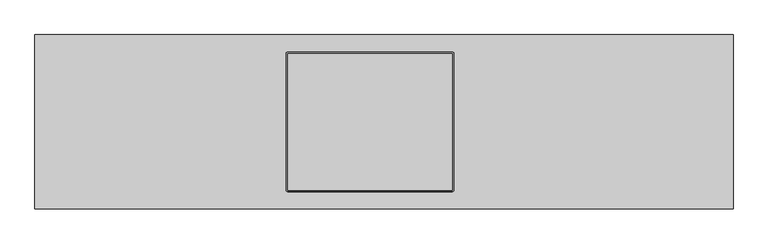
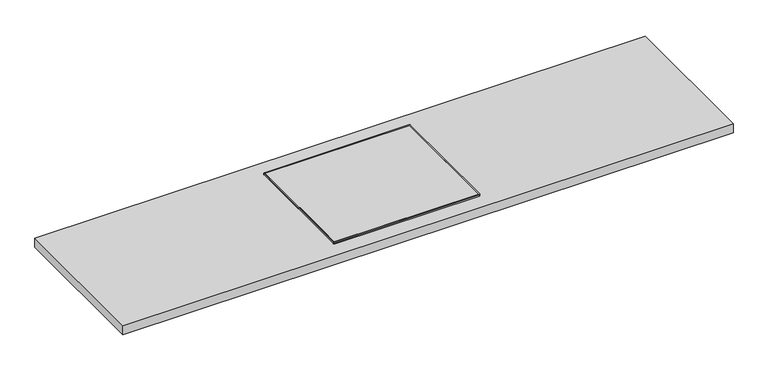
"""IFC4 building model written with IfcOpenShell, lengths in millimetres: furniture geometry, Arbeitsplatte - Mit Kochfeld : 600 mm Tiefe."""

from ifc_helpers import new_model, si_unit, point, frame, frame_2d, origin, place, context, project, spatial, polyline, circle_curve, trimmed, segment, composite_curve, outline, extrude, source, transform, mapped, element, save


def furniture_a2ae4300(model_context):
    return source(origin(), model_context, "Body", "SweptSolid", [
        extrude(outline(polyline([(294.5377049, -67.5), (294.5377049, -557.5), (-295.4622951, -557.5), (-295.4622951, -67.5), (294.5377049, -67.5)])), frame((0.0, 0.0, 900.0), z_axis=(0.0, 0.0, 1.0), x_axis=(1.0, 0.0, 0.0)), (0.0, 0.0, 1.0), 5.0),
        extrude(outline(composite_curve([segment(polyline([(-300.4622951, -557.5), (-300.4622951, -67.5)]), True, "CONTINUOUS"), segment(trimmed(circle_curve(frame_2d((-295.4622951, -67.5)), 5.0), [point((-300.4622951, -67.5))], [point((-295.4622951, -62.5))], False, "CARTESIAN"), True, "CONTINUOUS"), segment(polyline([(-295.4622951, -62.5), (294.5377049, -62.5)]), True, "CONTINUOUS"), segment(trimmed(circle_curve(frame_2d((294.5377049, -67.5)), 5.0), [point((294.5377049, -62.5))], [point((299.5377049, -67.5))], False, "CARTESIAN"), True, "CONTINUOUS"), segment(polyline([(299.5377049, -67.5), (299.5377049, -557.5)]), True, "CONTINUOUS"), segment(trimmed(circle_curve(frame_2d((294.5377049, -557.5)), 5.0), [point((299.5377049, -557.5))], [point((294.5377049, -562.5))], False, "CARTESIAN"), True, "CONTINUOUS"), segment(polyline([(294.5377049, -562.5), (-295.4622951, -562.5)]), True, "CONTINUOUS"), segment(trimmed(circle_curve(frame_2d((-295.4622951, -557.5)), 5.0), [point((-295.4622951, -562.5))], [point((-300.4622951, -557.5))], False, "CARTESIAN"), True, "CONTINUOUS")], self_intersect=False), holes=[polyline([(294.5377049, -67.5), (-295.4622951, -67.5), (-295.4622951, -557.5), (294.5377049, -557.5), (294.5377049, -67.5)])]), frame((0.0, 0.0, 900.0), z_axis=(0.0, 0.0, 1.0), x_axis=(1.0, 0.0, 0.0)), (0.0, 0.0, 1.0), 5.0),
        extrude(outline(polyline([(1299.5377049, 0.0), (1299.5377049, -625.0), (-1200.4622951, -625.0), (-1200.4622951, 0.0), (1299.5377049, 0.0)]), holes=[composite_curve([segment(polyline([(294.5377049, -62.5), (-295.4622951, -62.5)]), True, "CONTINUOUS"), segment(trimmed(circle_curve(frame_2d((-295.4622951, -67.5)), 5.0), [point((-295.4622951, -62.5))], [point((-300.4622951, -67.5))], True, "CARTESIAN"), True, "CONTINUOUS"), segment(polyline([(-300.4622951, -67.5), (-300.4622951, -557.5)]), True, "CONTINUOUS"), segment(trimmed(circle_curve(frame_2d((-295.4622951, -557.5)), 5.0), [point((-300.4622951, -557.5))], [point((-295.4622951, -562.5))], True, "CARTESIAN"), True, "CONTINUOUS"), segment(polyline([(-295.4622951, -562.5), (294.5377049, -562.5)]), True, "CONTINUOUS"), segment(trimmed(circle_curve(frame_2d((294.5377049, -557.5)), 5.0), [point((294.5377049, -562.5))], [point((299.5377049, -557.5))], True, "CARTESIAN"), True, "CONTINUOUS"), segment(polyline([(299.5377049, -557.5), (299.5377049, -67.5)]), True, "CONTINUOUS"), segment(trimmed(circle_curve(frame_2d((294.5377049, -67.5)), 5.0), [point((299.5377049, -67.5))], [point((294.5377049, -62.5))], True, "CARTESIAN"), True, "CONTINUOUS")], self_intersect=False)]), frame((0.0, 0.0, 860.0), z_axis=(0.0, 0.0, 1.0), x_axis=(1.0, 0.0, 0.0)), (0.0, 0.0, 1.0), 40.0),
    ])


if __name__ == "__main__":
    model = new_model("IFC4")
    model_context = context("Model", 3, world=origin())
    ifc_project = project(units=[si_unit("LENGTHUNIT", "METRE", prefix="MILLI")], contexts=[model_context])
    site = spatial("IfcSite", under=ifc_project)
    building = spatial("IfcBuilding", under=site)
    placement = place(None, origin())
    furniture_shape = furniture_a2ae4300(model_context)
    element("IfcFurniture", 1, ObjectType="Arbeitsplatte - Mit Kochfeld : 600 mm Tiefe", at=placement, inside=building, context=model_context, shape_type="MappedRepresentation", body=[
        mapped(furniture_shape, transform((0.0, 0.0, 0.0), x_axis=(1.0, 0.0, 0.0), y_axis=(0.0, 1.0, 0.0), z_axis=(0.0, 0.0, 1.0))),
    ])
    save(model, "model.ifc")

# Revit data of these elements
# Type "Arbeitsplatte - Mit Kochfeld : 600 mm Tiefe"
#   Dicke = 0.040 m
#   Depth = 0.625 m
#   Height = 0.900 m
#   Länge [instance default] = 2.500 m
#   Seitlicher Versatz Kochfeld [instance default] = 1.200 m
#   Tiefe Kochfeld [instance default] = 0.500 m
#   Breite Kochfeld [instance default] = 0.600 m
#   Rahmen Kochfeld = Metall - Aluminium
#   Kochfeld = Metall - Grau
#   Arbeitsplatte = Metall - Aluminium
# Element 1 (IfcFurniture, "Arbeitsplatte - Mit Kochfeld : 600 mm Tiefe")
#   Materials on its faces: "Metall - Aluminium", "Metall - Grau"
# Materials
#   "Metall - Aluminium": class "Metall", colour RGB 247 247 247, transparency 0, Description = "Aluminium 6061", Cost = 0
#   "Metall - Grau": class "Metall", colour RGB 60 60 60, transparency 0
